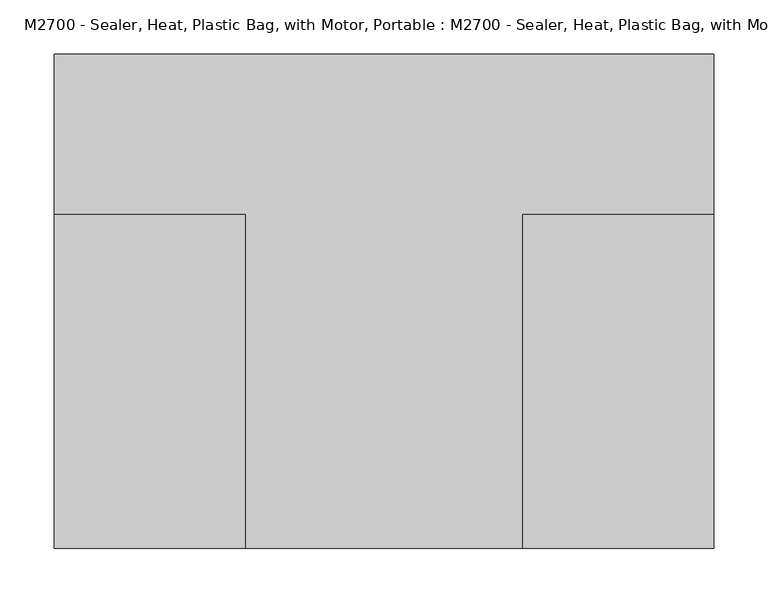
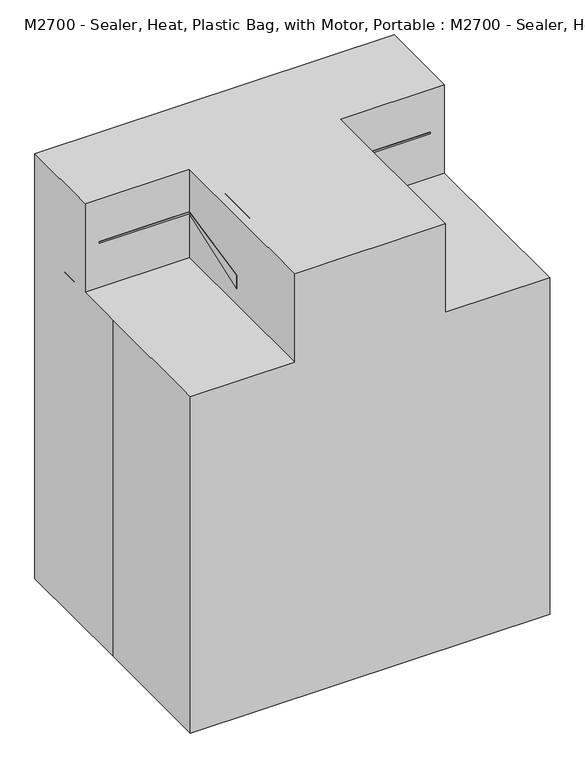
"""IFC4 building model written with IfcOpenShell, lengths in millimetres: proxy geometry, M2700 - Sealer, Heat, Plastic Bag, with Motor, Portable : M2700 - Sealer, Heat, Plastic Bag, with Motor, Portable."""

import ifcopenshell
import ifcopenshell.guid

model = None  # the IFC model being written
_history = None  # IfcOwnerHistory: only IFC2X3 demands one
_inside = {}  # id of a spatial element -> (the spatial element, [elements in it])
_under = {}  # id of a project, library or spatial element -> (it, [spatial elements below it])
_declared = {}  # id of a project -> (the project, [libraries it declares])
_typed = {}  # id of a type object -> (the type object, [elements of that type])
_made_of = {}  # id of a material, layer set ... -> (it, [elements and type objects made of it])


def new_model(schema):
    """Start an empty IFC model of exactly this schema.

    Asked for "IFC4X3", IfcOpenShell would pick the latest addendum, in which some entities
    have other attributes; the version numbers below select the first issue.
    IFC2X3 requires an IfcOwnerHistory on every rooted entity: one is made here for all.
    """
    global model, _history
    if schema == "IFC4X3":
        model = ifcopenshell.file(schema_version=(4, 3, 0, 0))
    else:
        model = ifcopenshell.file(schema=schema)
    _inside.clear()
    _under.clear()
    _declared.clear()
    _typed.clear()
    _made_of.clear()
    _history = None
    if model.schema == "IFC2X3":
        org = make("IfcOrganization", Name="unknown")
        user = make(
            "IfcPersonAndOrganization",
            ThePerson=make("IfcPerson", FamilyName="unknown"),
            TheOrganization=org,
        )
        app = make(
            "IfcApplication",
            ApplicationDeveloper=org,
            Version="unknown",
            ApplicationFullName="unknown",
            ApplicationIdentifier="unknown",
        )
        _history = make(
            "IfcOwnerHistory",
            OwningUser=user,
            OwningApplication=app,
            ChangeAction="ADDED",
            CreationDate=0,
        )
    return model


def make(cls, **values):
    """One entity of the class cls with the attributes given. An attribute that is None is left unset."""
    return model.create_entity(
        cls, **{name: value for name, value in values.items() if value is not None}
    )


def rooted(cls, **values):
    """An entity with a GlobalId (a new one), such as an element, a storey or a relation."""
    return make(cls, GlobalId=ifcopenshell.guid.new(), OwnerHistory=_history, **values)


def si_unit(unit_type, name, prefix=None):
    """IfcSIUnit, for example si_unit("LENGTHUNIT", "METRE", prefix="MILLI")."""
    return make("IfcSIUnit", UnitType=unit_type, Prefix=prefix, Name=name)


def assignment(units):
    """IfcUnitAssignment: the units of a project."""
    return None if units is None else make("IfcUnitAssignment", Units=units)


def point(xyz):
    """IfcCartesianPoint."""
    return None if xyz is None else make("IfcCartesianPoint", Coordinates=xyz)


def direction(xyz):
    """IfcDirection."""
    return None if xyz is None else make("IfcDirection", DirectionRatios=xyz)


def frame(location, z_axis=None, x_axis=None):
    """IfcAxis2Placement3D, a coordinate frame: its origin and axes. An axis left out is left unset."""
    return make(
        "IfcAxis2Placement3D",
        Location=point(location),
        Axis=direction(z_axis),
        RefDirection=direction(x_axis),
    )


def frame_2d(location, x_axis=None):
    """IfcAxis2Placement2D, a coordinate frame in the plane: its origin and x axis."""
    return make(
        "IfcAxis2Placement2D", Location=point(location), RefDirection=direction(x_axis)
    )


def origin():
    """The frame at (0, 0, 0) with its axes left unset."""
    return frame((0.0, 0.0, 0.0))


def origin_with_axes():
    """The frame at (0, 0, 0) with the z axis (0, 0, 1) and the x axis (1, 0, 0) written out."""
    return frame((0.0, 0.0, 0.0), z_axis=(0.0, 0.0, 1.0), x_axis=(1.0, 0.0, 0.0))


def place(relative_to, where):
    """IfcLocalPlacement: puts the frame where relative to a parent placement (None: the world)."""
    return make(
        "IfcLocalPlacement", PlacementRelTo=relative_to, RelativePlacement=where
    )


def context(
    kind, dimensions, precision=None, world=None, true_north=None, identifier=None
):
    """IfcGeometricRepresentationContext, for example the 3D "Model" context."""
    return make(
        "IfcGeometricRepresentationContext",
        ContextIdentifier=identifier,
        ContextType=kind,
        CoordinateSpaceDimension=dimensions,
        Precision=precision,
        WorldCoordinateSystem=world,
        TrueNorth=true_north,
    )


def project(units=None, contexts=None):
    """IfcProject with its units and contexts."""
    return rooted(
        "IfcProject",
        Name="project",
        RepresentationContexts=contexts,
        UnitsInContext=assignment(units),
    )


def spatial(cls, under=None, at=None, **own):
    """A site, building, storey or space (cls), placed at a placement, below another one or the project."""
    s = rooted(cls, ObjectPlacement=at, **own)
    if under is not None:
        _under.setdefault(under.id(), (under, []))[1].append(s)
    return s


def polyline(points):
    """IfcPolyline through the points."""
    return make("IfcPolyline", Points=[point(p) for p in points])


def circle_curve(where, radius):
    """IfcCircle in the frame where."""
    return make("IfcCircle", Position=where, Radius=radius)


def trimmed(basis, trim1, trim2, sense, master):
    """IfcTrimmedCurve: the piece of a basis curve between two trims."""
    return make(
        "IfcTrimmedCurve",
        BasisCurve=basis,
        Trim1=trim1,
        Trim2=trim2,
        SenseAgreement=sense,
        MasterRepresentation=master,
    )


def segment(curve, same_sense, transition):
    """IfcCompositeCurveSegment."""
    return make(
        "IfcCompositeCurveSegment",
        Transition=transition,
        SameSense=same_sense,
        ParentCurve=curve,
    )


def composite_curve(segments, self_intersect=None):
    """IfcCompositeCurve: segments joined end to end."""
    return make("IfcCompositeCurve", Segments=segments, SelfIntersect=self_intersect)


def outline(outer, holes=None, kind="AREA"):
    """IfcArbitraryClosedProfileDef: a profile drawn as a closed curve; with holes, ...WithVoids."""
    if holes is None:
        return make("IfcArbitraryClosedProfileDef", ProfileType=kind, OuterCurve=outer)
    return make(
        "IfcArbitraryProfileDefWithVoids",
        ProfileType=kind,
        OuterCurve=outer,
        InnerCurves=holes,
    )


def extrude(swept, where, along, depth):
    """IfcExtrudedAreaSolid: the profile swept, set in the frame where, extruded along a direction by depth."""
    return make(
        "IfcExtrudedAreaSolid",
        SweptArea=swept,
        Position=where,
        ExtrudedDirection=direction(along),
        Depth=depth,
    )


def faces_of(points, faces, orient=None, outer=None):
    """IfcFace entities. A face is a list of loops; a loop is a list of indices into points, from 0.

    orient and outer hold one flag for each loop. By default every Orientation is true, the
    first loop of a face is its IfcFaceOuterBound and the others are IfcFaceBound.
    """
    made = []
    for i, loops in enumerate(faces):
        bounds = []
        for j, loop in enumerate(loops):
            is_outer = j == 0 if outer is None else outer[i][j]
            bounds.append(
                make(
                    "IfcFaceOuterBound" if is_outer else "IfcFaceBound",
                    Bound=make("IfcPolyLoop", Polygon=[points[k] for k in loop]),
                    Orientation=True if orient is None else orient[i][j],
                )
            )
        made.append(make("IfcFace", Bounds=bounds))
    return made


def faceted_brep(points, faces, orient=None, outer=None, voids=None):
    """IfcFacetedBrep: a solid bounded by flat faces; with voids (closed shells), ...WithVoids."""
    shared = [point(p) for p in points]
    hull = make("IfcClosedShell", CfsFaces=faces_of(shared, faces, orient, outer))
    if voids is None:
        return make("IfcFacetedBrep", Outer=hull)
    return make(
        "IfcFacetedBrepWithVoids",
        Outer=hull,
        Voids=[
            make(cls, CfsFaces=faces_of(shared, fs, o, b)) for cls, fs, o, b in voids
        ],
    )


def shape(context_of_items, identifier, shape_type, items):
    """IfcShapeRepresentation: the items that make up one representation, for example the "Body"."""
    return make(
        "IfcShapeRepresentation",
        ContextOfItems=context_of_items,
        RepresentationIdentifier=identifier,
        RepresentationType=shape_type,
        Items=items,
    )


def source(mapping_origin, context_of_items, identifier, shape_type, items):
    """IfcRepresentationMap: a shape defined once, which mapped items show again and again."""
    return make(
        "IfcRepresentationMap",
        MappingOrigin=mapping_origin,
        MappedRepresentation=shape(context_of_items, identifier, shape_type, items),
    )


def transform(
    local_origin,
    x_axis=None,
    y_axis=None,
    z_axis=None,
    scale=None,
    scale2=None,
    scale3=None,
    uniform=True,
):
    """IfcCartesianTransformationOperator3D, or its non-uniform kind. x_axis, y_axis, z_axis: its Axis1, 2, 3."""
    if uniform:
        return make(
            "IfcCartesianTransformationOperator3D",
            Axis1=direction(x_axis),
            Axis2=direction(y_axis),
            LocalOrigin=point(local_origin),
            Scale=scale,
            Axis3=direction(z_axis),
        )
    return make(
        "IfcCartesianTransformationOperator3DnonUniform",
        Axis1=direction(x_axis),
        Axis2=direction(y_axis),
        LocalOrigin=point(local_origin),
        Scale=scale,
        Axis3=direction(z_axis),
        Scale2=scale2,
        Scale3=scale3,
    )


def mapped(mapping_source, mapping_target):
    """IfcMappedItem: shows the shape of a source again, moved by a transform."""
    return make(
        "IfcMappedItem", MappingSource=mapping_source, MappingTarget=mapping_target
    )


def made_of(thing, what):
    """Note that an element or type object is made of a material, layer set ...; save() writes the relation."""
    if what is not None:
        _made_of.setdefault(what.id(), (what, []))[1].append(thing)
    return thing


def element(
    cls,
    number,
    at=None,
    inside=None,
    cuts=None,
    type_object=None,
    material=None,
    context=None,
    identifier="Body",
    shape_type=None,
    held_by="IfcProductDefinitionShape",
    body=None,
    shapes=None,
    **own,
):
    """One element of the class cls, such as IfcWall. Its Tag is "e" and its number.

    at: its placement. inside: the storey or other place that contains it. cuts: it is an
    opening in that element (IfcRelVoidsElement). A single representation is given by context,
    identifier, shape_type and body (its items); several are given by shapes. held_by: the class
    of the entity that holds the representations. save() writes the other relations.
    """
    e = rooted(cls, Tag="e%d" % number, ObjectPlacement=at, **own)
    if body is not None:
        shapes = [shape(context, identifier, shape_type, body)]
    if shapes is not None:
        e.Representation = make(held_by, Representations=shapes)
    if inside is not None:
        _inside.setdefault(inside.id(), (inside, []))[1].append(e)
    if cuts is not None:
        rooted(
            "IfcRelVoidsElement", RelatingBuildingElement=cuts, RelatedOpeningElement=e
        )
    if type_object is not None:
        _typed.setdefault(type_object.id(), (type_object, []))[1].append(e)
    return made_of(e, material)


def aggregate(whole, parts):
    """IfcRelAggregates: a whole, such as a stair, and the parts it consists of."""
    return rooted("IfcRelAggregates", RelatingObject=whole, RelatedObjects=parts)


def save(model, path):
    """Write the relations noted so far, then the file.

    IfcRelAggregates (storeys below a building ...), IfcRelContainedInSpatialStructure (elements
    in a storey), IfcRelDefinesByType, IfcRelAssociatesMaterial and IfcRelDeclares: one each for
    every whole, place, type object, material and project.
    """
    for whole, parts in _under.values():
        aggregate(whole, parts)
    for where, things in _inside.values():
        rooted(
            "IfcRelContainedInSpatialStructure",
            RelatedElements=things,
            RelatingStructure=where,
        )
    for kind, things in _typed.values():
        rooted("IfcRelDefinesByType", RelatedObjects=things, RelatingType=kind)
    for what, things in _made_of.values():
        rooted("IfcRelAssociatesMaterial", RelatedObjects=things, RelatingMaterial=what)
    for by, libraries in _declared.values():
        rooted("IfcRelDeclares", RelatingContext=by, RelatedDefinitions=libraries)
    model.write(path)


def m2700_sealer_heat_plastic_bag_with_motor_portable_m2700_154b49e9(model_context):
    return source(origin(), model_context, "Body", "SolidModel", [
        extrude(outline(composite_curve([segment(trimmed(circle_curve(frame_2d((0.0, -12.7)), 12.7), [point((0.0, -25.4))], [point((0.0, 0.0))], False, "CARTESIAN"), True, "CONTINUOUS"), segment(trimmed(circle_curve(frame_2d((0.0, -12.7)), 12.7), [point((0.0, 0.0))], [point((0.0, -25.4))], False, "CARTESIAN"), True, "CONTINUOUS")], self_intersect=False)), frame((12.7, 15.9566276, 701.1420918), z_axis=(0.0, 0.7071067811865469, 0.7071067811865482), x_axis=(0.0, -0.7071067811865482, 0.7071067811865469)), (0.0, 0.0, 1.0), 43.6950974),
        faceted_brep([(280.8460579, 90.6708297, 685.9875921), (280.8460579, 90.6708297, 679.6375921), (280.8460579, 141.4708297, 679.6375921), (280.8460579, 141.4708297, 698.6875921), (280.8460579, 80.8223051, 685.7963503), (280.8460579, 80.8223051, 682.4030223), (-280.5077177, 141.4708297, 698.6875921), (-280.5077177, 141.4708297, 679.6375921), (-280.5077177, 90.6708297, 679.6375921), (-280.5077177, 90.6708297, 685.9875921), (-280.5077177, 80.8223051, 682.4030223), (-280.5077177, 80.8223051, 685.7963503), (-127.7852068, 80.8223051, 685.7963503), (-127.7852068, -58.5191973, 656.1783996), (127.7852068, -58.5191973, 656.1783996), (127.7852068, 80.8223051, 685.7963503), (-127.7852068, -58.5191973, 631.686863), (127.7852068, -58.5191973, 631.686863), (127.7852068, 80.8223051, 682.4030223), (-127.7852068, 80.8223051, 682.4030223)], [[[0, 1, 2, 3, 4, 5]], [[6, 7, 8, 9, 10, 11]], [[3, 6, 11, 12, 13, 14, 15, 4]], [[13, 16, 17, 14]], [[9, 0, 5, 18, 17, 16, 19, 10]], [[1, 0, 9, 8]], [[2, 1, 8, 7]], [[3, 2, 7, 6]], [[19, 12, 11, 10]], [[12, 19, 16, 13]], [[15, 18, 5, 4]], [[18, 15, 14, 17]]]),
        extrude(outline(composite_curve([segment(trimmed(circle_curve(frame_2d((101.6, -130.3161106)), 25.4), [point((127.0, -130.3161106))], [point((101.6, -155.7161106))], False, "CARTESIAN"), True, "CONTINUOUS"), segment(polyline([(101.6, -155.7161106), (73.025, -155.7161106)]), True, "CONTINUOUS"), segment(trimmed(circle_curve(frame_2d((73.025, -143.0161106)), 12.7), [point((73.025, -155.7161106))], [point((60.325, -143.0161106))], False, "CARTESIAN"), True, "CONTINUOUS"), segment(polyline([(60.325, -143.0161106), (60.325, -16.3922681)]), True, "CONTINUOUS"), segment(trimmed(circle_curve(frame_2d((41.275, -16.3922681)), 19.05), [point((60.325, -16.3922681))], [point((41.275, 2.6577319))], True, "CARTESIAN"), True, "CONTINUOUS"), segment(polyline([(41.275, 2.6577319), (-3.175, 2.6577319), (-47.625, 2.6577319)]), True, "CONTINUOUS"), segment(trimmed(circle_curve(frame_2d((-47.625, -16.3922681)), 19.05), [point((-47.625, 2.6577319))], [point((-66.675, -16.3922681))], True, "CARTESIAN"), True, "CONTINUOUS"), segment(polyline([(-66.675, -16.3922681), (-66.675, -142.2405353)]), True, "CONTINUOUS"), segment(trimmed(circle_curve(frame_2d((-79.375, -142.2405353)), 12.7), [point((-66.675, -142.2405353))], [point((-79.375, -154.9405353))], False, "CARTESIAN"), True, "CONTINUOUS"), segment(polyline([(-79.375, -154.9405353), (-102.3852068, -154.9405353)]), True, "CONTINUOUS"), segment(trimmed(circle_curve(frame_2d((-102.3852068, -129.5405353)), 25.4), [point((-102.3852068, -154.9405353))], [point((-127.7852068, -129.5405353))], False, "CARTESIAN"), True, "CONTINUOUS"), segment(polyline([(-127.7852068, -129.5405353), (-127.7852068, 55.4223051)]), True, "CONTINUOUS"), segment(trimmed(circle_curve(frame_2d((-102.3852068, 55.4223051)), 25.4), [point((-127.7852068, 55.4223051))], [point((-102.3852068, 80.8223051))], False, "CARTESIAN"), True, "CONTINUOUS"), segment(polyline([(-102.3852068, 80.8223051), (101.6, 80.8223051)]), True, "CONTINUOUS"), segment(trimmed(circle_curve(frame_2d((101.6, 55.4223051)), 25.4), [point((101.6, 80.8223051))], [point((127.0, 55.4223051))], False, "CARTESIAN"), True, "CONTINUOUS"), segment(polyline([(127.0, 55.4223051), (127.0, -130.3161106)]), True, "CONTINUOUS")], self_intersect=False)), frame((0.0, 0.0, 30.5919118), z_axis=(0.0, 0.0, 1.0), x_axis=(1.0, 0.0, 0.0)), (0.0, 0.0, 1.0), 27.2782251),
        extrude(outline(composite_curve([segment(polyline([(-203.2, -149.4929242), (-203.2, 93.6139601)]), True, "CONTINUOUS"), segment(trimmed(circle_curve(frame_2d((-190.5, 93.6139601)), 12.7), [point((-203.2, 93.6139601))], [point((-180.4752268, 101.4110059))], False, "CARTESIAN"), True, "CONTINUOUS"), segment(polyline([(-180.4752268, 101.4110059), (-116.8536353, 19.6118168)]), True, "CONTINUOUS"), segment(trimmed(circle_curve(frame_2d((-76.7545427, 50.8)), 50.8), [point((-116.8536353, 19.6118168))], [point((-76.7545427, 0.0))], True, "CARTESIAN"), True, "CONTINUOUS"), segment(polyline([(-76.7545427, 0.0), (76.7545427, 0.0)]), True, "CONTINUOUS"), segment(trimmed(circle_curve(frame_2d((76.7545427, 50.8)), 50.8), [point((76.7545427, 0.0))], [point((116.8536353, 19.6118168))], True, "CARTESIAN"), True, "CONTINUOUS"), segment(polyline([(116.8536353, 19.6118168), (180.4752268, 101.4110059)]), True, "CONTINUOUS"), segment(trimmed(circle_curve(frame_2d((190.5, 93.6139601)), 12.7), [point((180.4752268, 101.4110059))], [point((203.2, 93.6139601))], False, "CARTESIAN"), True, "CONTINUOUS"), segment(polyline([(203.2, 93.6139601), (203.2, -149.4929242)]), True, "CONTINUOUS"), segment(trimmed(circle_curve(frame_2d((190.5, -149.4929242)), 12.7), [point((203.2, -149.4929242))], [point((183.1182749, -159.8273392))], False, "CARTESIAN"), True, "CONTINUOUS"), segment(polyline([(183.1182749, -159.8273392), (176.1159248, -154.8256606)]), True, "CONTINUOUS"), segment(trimmed(circle_curve(frame_2d((10.027111, -387.35)), 285.75), [point((176.1159248, -154.8256606))], [point((10.027111, -101.6))], True, "CARTESIAN"), True, "CONTINUOUS"), segment(polyline([(10.027111, -101.6), (-10.027111, -101.6)]), True, "CONTINUOUS"), segment(trimmed(circle_curve(frame_2d((-10.027111, -387.35)), 285.75), [point((-10.027111, -101.6))], [point((-176.1159248, -154.8256606))], True, "CARTESIAN"), True, "CONTINUOUS"), segment(polyline([(-176.1159248, -154.8256606), (-183.1182749, -159.8273392)]), True, "CONTINUOUS"), segment(trimmed(circle_curve(frame_2d((-190.5, -149.4929242)), 12.7), [point((-183.1182749, -159.8273392))], [point((-203.2, -149.4929242))], False, "CARTESIAN"), True, "CONTINUOUS")], self_intersect=False)), origin_with_axes(), (0.0, 0.0, 1.0), 30.5919118),
        faceted_brep([(304.8, 228.6, 762.0), (-304.8, 228.6, 762.0), (-304.8, 80.8223051, 762.0), (-127.7852068, 80.8223051, 762.0), (-127.7852068, -228.6, 762.0), (127.7852068, -228.6, 762.0), (127.7852068, 80.8223051, 762.0), (304.8, 80.8223051, 762.0), (-304.8, 228.6, 0.0), (304.8, 228.6, 0.0), (304.8, -228.6, 0.0), (-304.8, -228.6, 0.0), (-304.8, 0.0, 0.0), (-304.8, 0.0, 603.4346392), (-304.8, 80.8223051, 603.4346392), (-304.8, -228.6, 603.4346392), (304.8, -228.6, 603.4346392), (127.7852068, -228.6, 603.4346392), (-127.7852068, -228.6, 603.4346392), (304.8, 80.8223051, 603.4346392), (-127.7852068, 80.8223051, 603.4346392), (127.7852068, 80.8223051, 603.4346392)], [[[0, 1, 2, 3, 4, 5, 6, 7]], [[8, 9, 10, 11, 12]], [[8, 12, 13, 14, 2, 1]], [[12, 11, 15, 13]], [[11, 10, 16, 17, 5, 4, 18, 15]], [[10, 9, 0, 7, 19, 16]], [[1, 0, 9, 8]], [[20, 14, 13, 15, 18]], [[14, 20, 3, 2]], [[20, 18, 4, 3]], [[21, 17, 16, 19]], [[21, 19, 7, 6]], [[17, 21, 6, 5]]]),
        extrude(outline(polyline([(603.25, 304.8), (603.25, 113.2371099), (603.25, -304.8), (577.85, -304.8), (577.85, 304.8), (603.25, 304.8)])), frame((0.0, 80.8223051, 0.0), z_axis=(0.0, 1.0, 0.0), x_axis=(0.0, 0.0, 1.0)), (0.0, 0.0, 1.0), 59.6394991),
        extrude(outline(composite_curve([segment(trimmed(circle_curve(frame_2d((0.0, -24.6438908)), 6.35), [point((-6.35, -24.6438908))], [point((6.35, -24.6438908))], False, "CARTESIAN"), True, "CONTINUOUS"), segment(trimmed(circle_curve(frame_2d((0.0, -24.6438908)), 6.35), [point((6.35, -24.6438908))], [point((-6.35, -24.6438908))], False, "CARTESIAN"), True, "CONTINUOUS")], self_intersect=False)), origin_with_axes(), (0.0, 0.0, 1.0), 603.4346392),
        extrude(outline(polyline([(-228.6, 603.4346392), (-228.6, 762.0), (0.0, 762.0), (80.8223051, 681.1776949), (80.8223051, 603.4346392), (-139.7, 603.4346392), (-228.6, 603.4346392)])), frame((-114.0497354, 0.0, 0.0), z_axis=(1.0, 0.0, 0.0), x_axis=(0.0, 1.0, 0.0)), (0.0, 0.0, 1.0), 227.2868453),
        extrude(outline(composite_curve([segment(trimmed(circle_curve(frame_2d((0.0, -101.6)), 38.1), [point((-38.1, -101.6))], [point((38.1, -101.6))], False, "CARTESIAN"), True, "CONTINUOUS"), segment(trimmed(circle_curve(frame_2d((0.0, -101.6)), 38.1), [point((38.1, -101.6))], [point((-38.1, -101.6))], False, "CARTESIAN"), True, "CONTINUOUS")], self_intersect=False)), origin_with_axes(), (0.0, 0.0, 1.0), 655.1196973),
        extrude(outline(composite_curve([segment(trimmed(circle_curve(frame_2d((0.0, -101.6)), 50.8), [point((-50.8, -101.6))], [point((50.8, -101.6))], False, "CARTESIAN"), True, "CONTINUOUS"), segment(trimmed(circle_curve(frame_2d((0.0, -101.6)), 50.8), [point((50.8, -101.6))], [point((-50.8, -101.6))], False, "CARTESIAN"), True, "CONTINUOUS")], self_intersect=False)), origin_with_axes(), (0.0, 0.0, 1.0), 75.0984896),
    ])


if __name__ == "__main__":
    model = new_model("IFC4")
    model_context = context("Model", 3, world=origin())
    ifc_project = project(units=[si_unit("LENGTHUNIT", "METRE", prefix="MILLI")], contexts=[model_context])
    site = spatial("IfcSite", under=ifc_project)
    building = spatial("IfcBuilding", under=site)
    placement = place(None, origin())
    m2700_sealer_heat_plastic_bag_with_motor_portable_m2700_shape = m2700_sealer_heat_plastic_bag_with_motor_portable_m2700_154b49e9(model_context)
    element("IfcBuildingElementProxy", 1, Name="M2700 - Sealer, Heat, Plastic Bag, with Motor, Portable : M2700 - Sealer, Heat, Plastic Bag, with Motor, Portable", ObjectType="M2700 - Sealer, Heat, Plastic Bag, with Motor, Portable : M2700 - Sealer, Heat, Plastic Bag, with Motor, Portable", at=placement, inside=building, context=model_context, shape_type="MappedRepresentation", body=[
        mapped(m2700_sealer_heat_plastic_bag_with_motor_portable_m2700_shape, transform((0.0, 0.0, 0.0), x_axis=(1.0, 0.0, 0.0), y_axis=(0.0, 1.0, 0.0), z_axis=(0.0, 0.0, 1.0))),
    ])
    save(model, "model.ifc")

# Revit data of these elements
# Type "M2700 - Sealer, Heat, Plastic Bag, with Motor, Portable : M2700 - Sealer, Heat, Plastic Bag, with Motor, Portable"
#   JSN = "M2700"
#   Nomenclature = "Sealer, Heat, Plastic Bag, w/Motor, Portable"
#   UTIL_2_Elec = "A"
#   Utility_6 = "-"
#   Utility_5 = "-"
#   Utility_4 = "-"
#   Utility_3 = "-"
#   Utility_2 = "A"
#   Utility_1 = "-"
#   Unit_Issue = "EA"
#   Price_Date = "0"
#   Nomenclature = "Sealer, Heat, Plastic Bag, w/Motor, Portable"
#   NSN = "3540"
#   Location [instance default] = ""
#   JSN_Name = "M2700"
#   Hertz_swit = "-1"
#   Hertz_dep = "-1"
#   Hertz = "60"
#   Desc = "Portable plastic bag heat sealing machine. Heavy duty portable sealer, motor driven with foot switch, 16 inches long clamping jaw minimum, 1/8 inch (2mm) wide heat seal, grounding plug and 3-wire electrical cable. Equipped with low voltage impulse generator with electronic timer. For making air and water-tight seals on plastic bags."
#   CAT_VA = "-"
#   CAT_Navy = "C"
#   CAT_IHS = "C"
#   CAT_Army = "C"
#   CAT_AF = "-"
#   BTUPerHour = "0"
#   Width_IN = 0
#   Weight_AV = 45
#   Watts2 = 0
#   Watts1 = 0
#   Volts2 = 0
#   Volts1 = 0
#   Phase2 = 0
#   Phase1 = 0
#   Height_IN = 0
#   Depth_IN = 0
#   Amps2 = 0
#   Amps1 = 0
# Element 1 (IfcBuildingElementProxy, "M2700 - Sealer, Heat, Plastic Bag, with Motor, Portable : M2700 - Sealer, Heat, Plastic Bag, with Motor, Portable")
#   Materials on its faces: "EquipSpace"
# Materials
#   "EquipSpace": class "Unassigned", colour RGB 221 217 195, transparency 0.5
